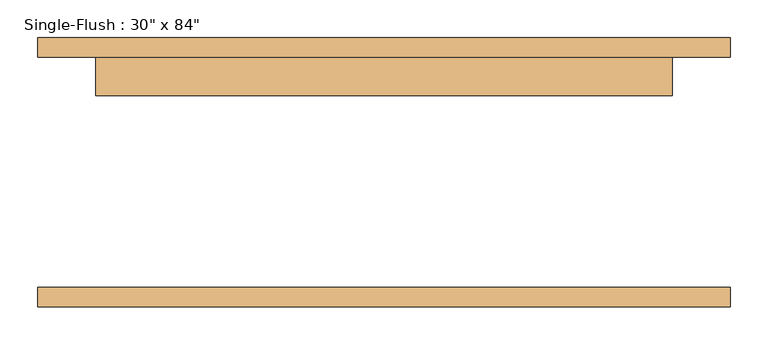
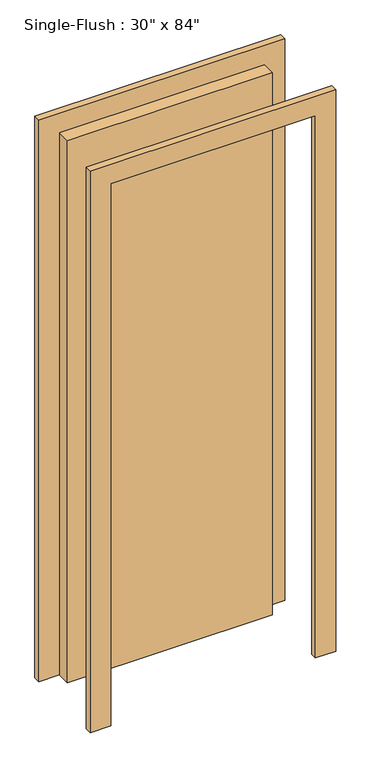
"""IFC4 building model written with IfcOpenShell, lengths in millimetres: door geometry."""

from ifc_helpers import new_model, si_unit, frame, origin, origin_with_axes, place, context, project, spatial, polyline, outline, extrude, source, transform, mapped, element, save


def door_fd98f027(model_context):
    return source(origin(), model_context, "Body", "SweptSolid", [
        extrude(outline(polyline([(2209.8, -457.2), (0.0, -457.2), (0.0, -381.0), (2133.6, -381.0), (2133.6, 381.0), (0.0, 381.0), (0.0, 457.2), (2209.8, 457.2), (2209.8, -457.2)])), frame((0.0, 152.4, 0.0), z_axis=(0.0, 1.0, 0.0), x_axis=(0.0, 0.0, 1.0)), (0.0, 0.0, 1.0), 25.4),
        extrude(outline(polyline([(2209.8, 457.2), (2209.8, -457.2), (0.0, -457.2), (0.0, -381.0), (2133.6, -381.0), (2133.6, 381.0), (0.0, 381.0), (0.0, 457.2), (2209.8, 457.2)])), frame((0.0, -177.8, 0.0), z_axis=(0.0, 1.0, 0.0), x_axis=(0.0, 0.0, 1.0)), (0.0, 0.0, 1.0), 25.4),
        extrude(outline(polyline([(381.0, 101.6), (-381.0, 101.6), (-381.0, 152.4), (381.0, 152.4), (381.0, 101.6)])), origin_with_axes(), (0.0, 0.0, 1.0), 2133.6),
    ])


if __name__ == "__main__":
    model = new_model("IFC4")
    model_context = context("Model", 3, world=origin())
    ifc_project = project(units=[si_unit("LENGTHUNIT", "METRE", prefix="MILLI")], contexts=[model_context])
    site = spatial("IfcSite", under=ifc_project)
    building = spatial("IfcBuilding", under=site)
    placement = place(None, origin())
    door_shape = door_fd98f027(model_context)
    element("IfcDoor", 1, ObjectType="Single-Flush : 30\" x 84\"", at=placement, inside=building, context=model_context, shape_type="MappedRepresentation", body=[
        mapped(door_shape, transform((0.0, 0.0, 0.0), x_axis=(1.0, 0.0, 0.0), y_axis=(0.0, 1.0, 0.0), z_axis=(0.0, 0.0, 1.0))),
    ])
    save(model, "model.ifc")

# Revit data of these elements
# Type "Single-Flush : 30\" x 84\""
#   Type Mark = "4"
#   Construction Type Id = "MDOOR"
#   Assembly Code = "C1020"
#   Analytic Construction = "Metal"
#   Thickness = 0' - 2"
#   Heat Transfer Coefficient (U) = 0.651978 BTU/(h·ft²·°F)
#   Height = 7' - 0"
#   Trim Projection Ext = 0' - 1"
#   Trim Projection Int = 0' - 1"
#   Trim Width = 0' - 3"
#   Width = 2' - 6"
#   Define Thermal Properties by = 1
#   Define Thermal Properties by = 1
#   Door Material = Door - Panel
#   Frame Material = Door - Frame
#   Visual Light Transmittance = 0
#   Solar Heat Gain Coefficient = 0
#   Function = (empty or 0)
#   Wall Closure = (empty or 0)
# Element 1 (IfcDoor, "Single-Flush : 30\" x 84\"")
#   Materials on its faces: "Door - Frame", "Door - Panel"
# Materials
#   "Door - Panel": class "Wood", colour RGB 210 159 95, transparency 0, Cost = 0
#   "Door - Frame": class "Miscellaneous", colour RGB 118 70 51, transparency 0, Cost = 0
